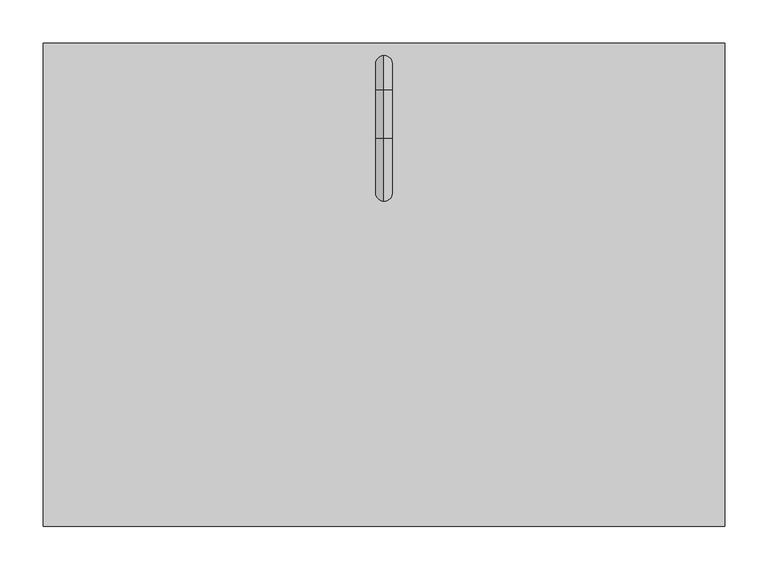
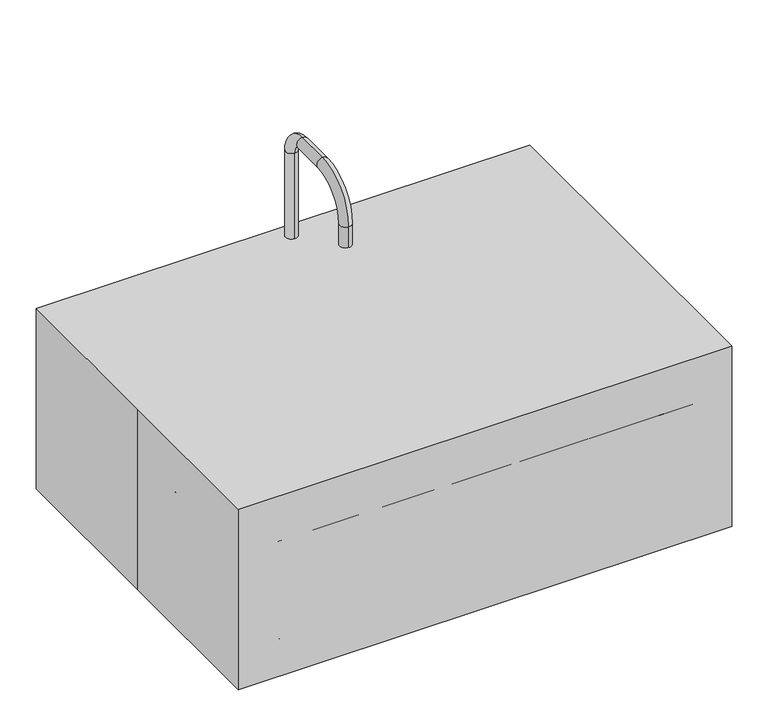
"""IFC4 building model written with IfcOpenShell, lengths in millimetres: proxy geometry, CS200 - Sink, SS, Single Compartment, 12x28x16 ID : CS200 - Sink, SS, Single Compartment, 12x28x16 ID."""

from ifc_helpers import new_model, si_unit, point, frame, frame_2d, origin, origin_with_axes, origin_2d, place, context, project, spatial, polyline, circle_curve, ellipse_curve, trimmed, segment, composite_curve, outline, extrude, source, transform, mapped, element, save
from ifc_brep_helpers import plane_surface, cylinder_surface, revolved_surface, advanced_brep


def specialty_equipment_f0ebf2b9(model_context):
    return source(origin(), model_context, "Body", "SolidModel", [
        extrude(outline(composite_curve([segment(trimmed(circle_curve(frame_2d((292.1, 168.275)), 25.4), [point((292.1, 193.675))], [point((317.5, 168.275))], False, "CARTESIAN"), True, "CONTINUOUS"), segment(polyline([(317.5, 168.275), (317.5, -177.8)]), True, "CONTINUOUS"), segment(trimmed(circle_curve(frame_2d((292.1, -177.8)), 25.4), [point((317.5, -177.8))], [point((292.1, -203.2))], False, "CARTESIAN"), True, "CONTINUOUS"), segment(polyline([(292.1, -203.2), (-292.1000001, -203.2)]), True, "CONTINUOUS"), segment(trimmed(circle_curve(frame_2d((-292.1000001, -177.8)), 25.4), [point((-292.1000001, -203.2))], [point((-317.5000001, -177.8))], False, "CARTESIAN"), True, "CONTINUOUS"), segment(polyline([(-317.5000001, -177.8), (-317.5000001, 168.275)]), True, "CONTINUOUS"), segment(trimmed(circle_curve(frame_2d((-292.1000001, 168.275)), 25.4), [point((-317.5000001, 168.275))], [point((-292.1000001, 193.675))], False, "CARTESIAN"), True, "CONTINUOUS"), segment(polyline([(-292.1000001, 193.675), (292.1, 193.675)]), True, "CONTINUOUS")], self_intersect=False), holes=[composite_curve([segment(trimmed(circle_curve(origin_2d(), 25.4), [point((-25.4, 0.0))], [point((25.4, 0.0))], True, "CARTESIAN"), True, "CONTINUOUS"), segment(trimmed(circle_curve(origin_2d(), 25.4), [point((25.4, 0.0))], [point((-25.4, 0.0))], True, "CARTESIAN"), True, "CONTINUOUS")], self_intersect=False)]), origin_with_axes(), (0.0, 0.0, 1.0), 9.525),
        extrude(outline(polyline([(-393.7, 279.4), (393.7, 279.4), (393.7, -279.4), (-393.7, -279.4), (-393.7, 0.0), (-393.7, 279.4)])), origin_with_axes(), (0.0, 0.0, 1.0), 304.8),
        extrude(outline(composite_curve([segment(trimmed(circle_curve(frame_2d((82.55, 260.35)), 19.05), [point((82.55, 279.4))], [point((82.55, 241.3))], False, "CARTESIAN"), True, "CONTINUOUS"), segment(polyline([(82.55, 241.3), (-82.55, 241.3)]), True, "CONTINUOUS"), segment(trimmed(circle_curve(frame_2d((-82.55, 260.35)), 19.05), [point((-82.55, 241.3))], [point((-82.55, 279.4))], False, "CARTESIAN"), True, "CONTINUOUS"), segment(polyline([(-82.55, 279.4), (82.55, 279.4)]), True, "CONTINUOUS")], self_intersect=False), holes=[composite_curve([segment(trimmed(circle_curve(frame_2d((0.0, 255.5875)), 9.525), [point((-9.525, 255.5875))], [point((9.525, 255.5875))], True, "CARTESIAN"), True, "CONTINUOUS"), segment(trimmed(circle_curve(frame_2d((0.0, 255.5875)), 9.525), [point((9.525, 255.5875))], [point((-9.525, 255.5875))], True, "CARTESIAN"), True, "CONTINUOUS")], self_intersect=False)]), frame((0.0, 0.0, 228.6), z_axis=(0.0, 0.0, 1.0), x_axis=(1.0, 0.0, 0.0)), (0.0, 0.0, 1.0), 12.7),
        extrude(outline(composite_curve([segment(trimmed(circle_curve(frame_2d((-1e-07, 255.5875)), 12.7), [point((-12.7000001, 255.5875))], [point((12.6999999, 255.5875))], False, "CARTESIAN"), True, "CONTINUOUS"), segment(trimmed(circle_curve(frame_2d((-1e-07, 255.5875)), 12.7), [point((12.6999999, 255.5875))], [point((-12.7000001, 255.5875))], False, "CARTESIAN"), True, "CONTINUOUS")], self_intersect=False), holes=[composite_curve([segment(trimmed(circle_curve(frame_2d((-1e-07, 255.5875)), 9.525), [point((-9.5250001, 255.5875))], [point((9.5249999, 255.5875))], True, "CARTESIAN"), True, "CONTINUOUS"), segment(trimmed(circle_curve(frame_2d((-1e-07, 255.5875)), 9.525), [point((9.5249999, 255.5875))], [point((-9.5250001, 255.5875))], True, "CARTESIAN"), True, "CONTINUOUS")], self_intersect=False)]), frame((0.0, 0.0, 241.3), z_axis=(0.0, 0.0, 1.0), x_axis=(1.0, 0.0, 0.0)), (0.0, 0.0, 1.0), 12.7),
        advanced_brep(
        [(-1e-07, 265.1125, 228.6), (-1e-07, 246.0625, 228.6), (-1e-07, 265.1125, 449.2625), (-1e-07, 246.0625, 449.2625), (-1e-07, 225.425, 469.9), (-1e-07, 225.425, 488.95), (-1e-07, 169.8625, 488.95), (-1e-07, 169.8625, 469.9), (-1e-07, 115.8875, 415.925), (-1e-07, 96.8375, 415.925), (-1e-07, 96.8375, 381.0), (-1e-07, 115.8875, 381.0)],
        [
            (0, 1, circle_curve(frame((-1e-07, 255.5875, 228.6), z_axis=(0.0, 0.0, -1.0), x_axis=(0.0, -1.0, 0.0)), 9.525)),
            (1, 0, circle_curve(frame((-1e-07, 255.5875, 228.6), z_axis=(0.0, 0.0, -1.0), x_axis=(0.0, -1.0, 0.0)), 9.525)),
            (0, 2),
            (2, 3, circle_curve(frame((-1e-07, 255.5875, 449.2625), z_axis=(0.0, 0.0, -1.0), x_axis=(0.0, -1.0, 0.0)), 9.525)),
            (3, 1),
            (3, 2, circle_curve(frame((-1e-07, 255.5875, 449.2625), z_axis=(0.0, 0.0, -1.0), x_axis=(0.0, -1.0, 0.0)), 9.525)),
            (4, 3, circle_curve(frame((-1e-07, 225.425, 449.2625), z_axis=(-1.0, 0.0, 0.0), x_axis=(0.0, 1.0, 0.0)), 20.6375)),
            (2, 5, circle_curve(frame((-1e-07, 225.425, 449.2625), z_axis=(1.0, 0.0, 0.0), x_axis=(0.0, 1.0, 0.0)), 39.6875)),
            (5, 4, circle_curve(frame((-1e-07, 225.425, 479.425), z_axis=(0.0, 1.0, 0.0), x_axis=(0.0, 0.0, -1.0)), 9.525)),
            (4, 5, circle_curve(frame((-1e-07, 225.425, 479.425), z_axis=(0.0, 1.0, 0.0), x_axis=(0.0, 0.0, -1.0)), 9.525)),
            (5, 6),
            (6, 7, circle_curve(frame((-1e-07, 169.8625, 479.425), z_axis=(0.0, 1.0, 0.0), x_axis=(0.0, 0.0, -1.0)), 9.525)),
            (7, 4),
            (7, 6, circle_curve(frame((-1e-07, 169.8625, 479.425), z_axis=(0.0, 1.0, 0.0), x_axis=(0.0, 0.0, -1.0)), 9.525)),
            (8, 7, circle_curve(frame((-1e-07, 169.8625, 415.925), z_axis=(-1.0, 0.0, 0.0), x_axis=(0.0, 0.0, 1.0)), 53.975)),
            (6, 9, circle_curve(frame((-1e-07, 169.8625, 415.925), z_axis=(1.0, 0.0, 0.0), x_axis=(0.0, 0.0, 1.0)), 73.025)),
            (9, 8, circle_curve(frame((-1e-07, 106.3625, 415.925), z_axis=(0.0, 0.0, 1.0), x_axis=(0.0, 1.0, 0.0)), 9.525)),
            (8, 9, circle_curve(frame((-1e-07, 106.3625, 415.925), z_axis=(0.0, 0.0, 1.0), x_axis=(0.0, 1.0, 0.0)), 9.525)),
            (10, 11, circle_curve(frame((-1e-07, 106.3625, 381.0), z_axis=(0.0, 0.0, -1.0), x_axis=(0.0, 1.0, 0.0)), 9.525)),
            (11, 10, circle_curve(frame((-1e-07, 106.3625, 381.0), z_axis=(0.0, 0.0, -1.0), x_axis=(0.0, 1.0, 0.0)), 9.525)),
            (9, 10),
            (11, 8),
        ],
        [
            plane_surface(frame((-1e-07, 246.0625, 228.6), z_axis=(0.0, 0.0, -1.0), x_axis=(1.0, 0.0, 0.0))),
            cylinder_surface(frame((-1e-07, 255.5875, 228.6), z_axis=(0.0, 0.0, -1.0), x_axis=(0.0, -1.0, 0.0)), 9.525),
            revolved_surface(trimmed(ellipse_curve(frame((-1e-07, 255.5875, 449.2625), z_axis=(0.0, 0.0, -1.0), x_axis=(0.0, -1.0, 0.0)), 9.525, 9.525), [point((-1e-07, 265.1125, 449.2625))], [point((-1e-07, 246.0625, 449.2625))], True, "CARTESIAN"), (-1e-07, 225.425, 449.2625), (1.0, 0.0, 0.0)),
            revolved_surface(trimmed(ellipse_curve(frame((-1e-07, 255.5875, 449.2625), z_axis=(0.0, 0.0, -1.0), x_axis=(0.0, -1.0, 0.0)), 9.525, 9.525), [point((-1e-07, 246.0625, 449.2625))], [point((-1e-07, 265.1125, 449.2625))], True, "CARTESIAN"), (-1e-07, 225.425, 449.2625), (1.0, 0.0, 0.0)),
            cylinder_surface(frame((-1e-07, 225.425, 479.425), z_axis=(0.0, 1.0, 0.0), x_axis=(0.0, 0.0, -1.0)), 9.525),
            revolved_surface(trimmed(ellipse_curve(frame((-1e-07, 169.8625, 479.425), z_axis=(0.0, 1.0, 0.0), x_axis=(0.0, 0.0, -1.0)), 9.525, 9.525), [point((-1e-07, 169.8625, 488.95))], [point((-1e-07, 169.8625, 469.9))], True, "CARTESIAN"), (-1e-07, 169.8625, 415.925), (1.0, 0.0, 0.0)),
            revolved_surface(trimmed(ellipse_curve(frame((-1e-07, 169.8625, 479.425), z_axis=(0.0, 1.0, 0.0), x_axis=(0.0, 0.0, -1.0)), 9.525, 9.525), [point((-1e-07, 169.8625, 469.9))], [point((-1e-07, 169.8625, 488.95))], True, "CARTESIAN"), (-1e-07, 169.8625, 415.925), (1.0, 0.0, 0.0)),
            plane_surface(frame((-1e-07, 96.8375, 381.0), z_axis=(0.0, 0.0, -1.0), x_axis=(-1.0, 0.0, 0.0))),
            cylinder_surface(frame((-1e-07, 106.3625, 415.925), z_axis=(0.0, 0.0, 1.0), x_axis=(0.0, 1.0, 0.0)), 9.525),
        ],
        [
            (0, [[1, 2]]),
            (1, [[-1, 3, 4, 5]]),
            (1, [[-2, -5, 6, -3]]),
            (2, [[7, -4, 8, 9]]),
            (3, [[-8, -6, -7, 10]]),
            (4, [[-9, 11, 12, 13]]),
            (4, [[-10, -13, 14, -11]]),
            (5, [[15, -12, 16, 17]]),
            (6, [[-16, -14, -15, 18]]),
            (7, [[19, 20]]),
            (8, [[-17, 21, -20, 22]]),
            (8, [[-18, -22, -19, -21]]),
        ],
    ),
        extrude(outline(composite_curve([segment(trimmed(circle_curve(frame_2d((-57.15, 260.35)), 19.05), [point((-76.2, 260.35))], [point((-38.1, 260.35))], False, "CARTESIAN"), True, "CONTINUOUS"), segment(trimmed(circle_curve(frame_2d((-57.15, 260.35)), 19.05), [point((-38.1, 260.35))], [point((-76.2, 260.35))], False, "CARTESIAN"), True, "CONTINUOUS")], self_intersect=False)), frame((0.0, 0.0, 241.3), z_axis=(0.0, 0.0, 1.0), x_axis=(1.0, 0.0, 0.0)), (0.0, 0.0, 1.0), 50.8),
        extrude(outline(composite_curve([segment(trimmed(circle_curve(frame_2d((57.15, 260.35)), 19.05), [point((38.1, 260.35))], [point((76.2, 260.35))], False, "CARTESIAN"), True, "CONTINUOUS"), segment(trimmed(circle_curve(frame_2d((57.15, 260.35)), 19.05), [point((76.2, 260.35))], [point((38.1, 260.35))], False, "CARTESIAN"), True, "CONTINUOUS")], self_intersect=False)), frame((0.0, 0.0, 241.3), z_axis=(0.0, 0.0, 1.0), x_axis=(1.0, 0.0, 0.0)), (0.0, 0.0, 1.0), 50.8),
        advanced_brep(
        [(-292.1000001, 238.125, 0.0), (-292.1000001, 238.125, 215.9), (292.1, 238.125, 215.9), (292.1, 238.125, 0.0), (-292.1000001, 193.675, 0.0), (292.1, 193.675, 0.0), (-292.1000001, 193.675, 9.525), (292.1, 193.675, 9.525), (-292.1000001, 196.2634182, 9.525), (292.1, 196.2634182, 9.525), (-292.1000001, 215.2409272, 26.9146831), (292.1, 215.2409272, 26.9146831), (-292.1000001, 231.775, 215.9), (292.1, 231.775, 215.9), (361.95, 168.275, 0.0), (361.95, 168.275, 215.9), (317.5, 168.275, 0.0), (317.5, 168.275, 9.525), (320.0884182, 168.275, 9.525), (339.0659272, 168.275, 26.9146831), (355.6, 168.275, 215.9), (361.95, -177.8, 215.9), (361.95, -177.8, 0.0), (317.5, -177.8, 0.0), (317.5, -177.8, 9.525), (320.0884182, -177.8, 9.525), (339.0659272, -177.8, 26.9146831), (355.6, -177.8, 215.9), (292.1, -247.65, 0.0), (292.1, -247.65, 215.9), (292.1, -203.2, 0.0), (292.1, -203.2, 9.525), (292.1, -205.7884182, 9.525), (292.1, -224.7659272, 26.9146831), (292.1, -241.3, 215.9), (-292.1000001, -247.65, 215.9), (-292.1000001, -247.65, 0.0), (-292.1000001, -203.2, 0.0), (-292.1000001, -203.2, 9.525), (-292.1000001, -205.7884182, 9.525), (-292.1000001, -224.7659272, 26.9146831), (-292.1000001, -241.3, 215.9), (-361.9500001, -177.8, 0.0), (-361.9500001, -177.8, 215.9), (-317.5000001, -177.8, 0.0), (-317.5000001, -177.8, 9.525), (-320.0884183, -177.8, 9.525), (-339.0659273, -177.8, 26.9146831), (-355.6000001, -177.8, 215.9), (-361.9500001, 168.275, 215.9), (-361.9500001, 168.275, 0.0), (-317.5000001, 168.275, 0.0), (-317.5000001, 168.275, 9.525), (-320.0884183, 168.275, 9.525), (-339.0659273, 168.275, 26.9146831), (-355.6000001, 168.275, 215.9)],
        [
            (0, 1),
            (1, 2),
            (2, 3),
            (3, 0),
            (4, 0),
            (3, 5),
            (5, 4),
            (6, 4),
            (5, 7),
            (7, 6),
            (8, 6),
            (7, 9),
            (9, 8),
            (10, 8, circle_curve(frame((-292.1000001, 196.2634182, 28.575), z_axis=(-1.0, 0.0, 0.0), x_axis=(0.0, 1.0, 0.0)), 19.05)),
            (9, 11, circle_curve(frame((292.1, 196.2634182, 28.575), z_axis=(1.0, 0.0, 0.0), x_axis=(0.0, 1.0, 0.0)), 19.05)),
            (11, 10),
            (12, 10),
            (11, 13),
            (13, 12),
            (1, 12),
            (13, 2),
            (14, 3, circle_curve(frame((292.1, 168.275, 0.0), z_axis=(0.0, 0.0, 1.0), x_axis=(0.0, 1.0, 0.0)), 69.85)),
            (2, 15, circle_curve(frame((292.1, 168.275, 215.9), z_axis=(0.0, 0.0, -1.0), x_axis=(0.0, 1.0, 0.0)), 69.85)),
            (15, 14),
            (16, 5, circle_curve(frame((292.1, 168.275, 0.0), z_axis=(0.0, 0.0, 1.0), x_axis=(0.0, 1.0, 0.0)), 25.4)),
            (14, 16),
            (17, 7, circle_curve(frame((292.1, 168.275, 9.525), z_axis=(0.0, 0.0, 1.0), x_axis=(0.0, 1.0, 0.0)), 25.4)),
            (16, 17),
            (18, 9, circle_curve(frame((292.1, 168.275, 9.525), z_axis=(0.0, 0.0, 1.0), x_axis=(0.0, 1.0, 0.0)), 27.9884182)),
            (17, 18),
            (19, 11, circle_curve(frame((292.1, 168.275, 26.9146831), z_axis=(0.0, 0.0, 1.0), x_axis=(0.0, 1.0, 0.0)), 46.9659272)),
            (18, 19, circle_curve(frame((320.0884182, 168.275, 28.575), z_axis=(0.0, -1.0, 0.0), x_axis=(1.0, 0.0, 0.0)), 19.05)),
            (20, 13, circle_curve(frame((292.1, 168.275, 215.9), z_axis=(0.0, 0.0, 1.0), x_axis=(0.0, 1.0, 0.0)), 63.5)),
            (19, 20),
            (20, 15),
            (15, 21),
            (21, 22),
            (22, 14),
            (22, 23),
            (23, 16),
            (23, 24),
            (24, 17),
            (24, 25),
            (25, 18),
            (25, 26, circle_curve(frame((320.0884182, -177.8, 28.575), z_axis=(0.0, -1.0, 0.0), x_axis=(1.0, 0.0, 0.0)), 19.05)),
            (26, 19),
            (26, 27),
            (27, 20),
            (27, 21),
            (28, 22, circle_curve(frame((292.1, -177.8, 0.0), z_axis=(0.0, 0.0, 1.0), x_axis=(1.0, 0.0, 0.0)), 69.85)),
            (21, 29, circle_curve(frame((292.1, -177.8, 215.9), z_axis=(0.0, 0.0, -1.0), x_axis=(1.0, 0.0, 0.0)), 69.85)),
            (29, 28),
            (30, 23, circle_curve(frame((292.1, -177.8, 0.0), z_axis=(0.0, 0.0, 1.0), x_axis=(1.0, 0.0, 0.0)), 25.4)),
            (28, 30),
            (31, 24, circle_curve(frame((292.1, -177.8, 9.525), z_axis=(0.0, 0.0, 1.0), x_axis=(1.0, 0.0, 0.0)), 25.4)),
            (30, 31),
            (32, 25, circle_curve(frame((292.1, -177.8, 9.525), z_axis=(0.0, 0.0, 1.0), x_axis=(1.0, 0.0, 0.0)), 27.9884182)),
            (31, 32),
            (33, 26, circle_curve(frame((292.1, -177.8, 26.9146831), z_axis=(0.0, 0.0, 1.0), x_axis=(1.0, 0.0, 0.0)), 46.9659272)),
            (32, 33, circle_curve(frame((292.1, -205.7884182, 28.575), z_axis=(-1.0, 0.0, 0.0), x_axis=(0.0, -1.0, 0.0)), 19.05)),
            (34, 27, circle_curve(frame((292.1, -177.8, 215.9), z_axis=(0.0, 0.0, 1.0), x_axis=(1.0, 0.0, 0.0)), 63.5)),
            (33, 34),
            (34, 29),
            (29, 35),
            (35, 36),
            (36, 28),
            (36, 37),
            (37, 30),
            (37, 38),
            (38, 31),
            (38, 39),
            (39, 32),
            (39, 40, circle_curve(frame((-292.1000001, -205.7884182, 28.575), z_axis=(-1.0, 0.0, 0.0), x_axis=(0.0, -1.0, 0.0)), 19.05)),
            (40, 33),
            (40, 41),
            (41, 34),
            (41, 35),
            (42, 36, circle_curve(frame((-292.1000001, -177.8, 0.0), z_axis=(0.0, 0.0, 1.0), x_axis=(0.0, -1.0, 0.0)), 69.85)),
            (35, 43, circle_curve(frame((-292.1000001, -177.8, 215.9), z_axis=(0.0, 0.0, -1.0), x_axis=(0.0, -1.0, 0.0)), 69.85)),
            (43, 42),
            (44, 37, circle_curve(frame((-292.1000001, -177.8, 0.0), z_axis=(0.0, 0.0, 1.0), x_axis=(0.0, -1.0, 0.0)), 25.4)),
            (42, 44),
            (45, 38, circle_curve(frame((-292.1000001, -177.8, 9.525), z_axis=(0.0, 0.0, 1.0), x_axis=(0.0, -1.0, 0.0)), 25.4)),
            (44, 45),
            (46, 39, circle_curve(frame((-292.1000001, -177.8, 9.525), z_axis=(0.0, 0.0, 1.0), x_axis=(0.0, -1.0, 0.0)), 27.9884182)),
            (45, 46),
            (47, 40, circle_curve(frame((-292.1000001, -177.8, 26.9146831), z_axis=(0.0, 0.0, 1.0), x_axis=(0.0, -1.0, 0.0)), 46.9659272)),
            (46, 47, circle_curve(frame((-320.0884183, -177.8, 28.575), z_axis=(0.0, 1.0, 0.0), x_axis=(-1.0, 0.0, 0.0)), 19.05)),
            (48, 41, circle_curve(frame((-292.1000001, -177.8, 215.9), z_axis=(0.0, 0.0, 1.0), x_axis=(0.0, -1.0, 0.0)), 63.5)),
            (47, 48),
            (48, 43),
            (43, 49),
            (49, 50),
            (50, 42),
            (50, 51),
            (51, 44),
            (51, 52),
            (52, 45),
            (52, 53),
            (53, 46),
            (53, 54, circle_curve(frame((-320.0884183, 168.275, 28.575), z_axis=(0.0, 1.0, 0.0), x_axis=(-1.0, 0.0, 0.0)), 19.05)),
            (54, 47),
            (54, 55),
            (55, 48),
            (55, 49),
            (0, 50, circle_curve(frame((-292.1000001, 168.275, 0.0), z_axis=(0.0, 0.0, 1.0), x_axis=(-1.0, 0.0, 0.0)), 69.85)),
            (49, 1, circle_curve(frame((-292.1000001, 168.275, 215.9), z_axis=(0.0, 0.0, -1.0), x_axis=(-1.0, 0.0, 0.0)), 69.85)),
            (4, 51, circle_curve(frame((-292.1000001, 168.275, 0.0), z_axis=(0.0, 0.0, 1.0), x_axis=(-1.0, 0.0, 0.0)), 25.4)),
            (6, 52, circle_curve(frame((-292.1000001, 168.275, 9.525), z_axis=(0.0, 0.0, 1.0), x_axis=(-1.0, 0.0, 0.0)), 25.4)),
            (8, 53, circle_curve(frame((-292.1000001, 168.275, 9.525), z_axis=(0.0, 0.0, 1.0), x_axis=(-1.0, 0.0, 0.0)), 27.9884182)),
            (10, 54, circle_curve(frame((-292.1000001, 168.275, 26.9146831), z_axis=(0.0, 0.0, 1.0), x_axis=(-1.0, 0.0, 0.0)), 46.9659272)),
            (12, 55, circle_curve(frame((-292.1000001, 168.275, 215.9), z_axis=(0.0, 0.0, 1.0), x_axis=(-1.0, 0.0, 0.0)), 63.5)),
        ],
        [
            plane_surface(frame((-292.1000001, 238.125, 215.9), z_axis=(0.0, 1.0, 0.0), x_axis=(1.0, 0.0, 0.0))),
            plane_surface(frame((-292.1000001, 238.125, 0.0), z_axis=(0.0, 0.0, -1.0), x_axis=(1.0, 0.0, 0.0))),
            plane_surface(frame((-292.1000001, 193.675, 0.0), z_axis=(0.0, -1.0, 0.0), x_axis=(1.0, 0.0, 0.0))),
            plane_surface(frame((-292.1000001, 193.675, 9.525), z_axis=(0.0, 0.0, 1.0), x_axis=(1.0, 0.0, 0.0))),
            revolved_surface(polyline([(292.1, 215.3134182, 28.575), (-292.1000001, 215.3134182, 28.575)]), (-292.1000001, 196.2634182, 28.575), (1.0, 0.0, 0.0)),
            plane_surface(frame((-292.1000001, 215.2409272, 26.9146831), z_axis=(0.0, -0.9961946980917442, 0.08715574274767357), x_axis=(1.0, 0.0, 0.0))),
            plane_surface(frame((-292.1000001, 231.775, 215.9), z_axis=(0.0, 0.0, 1.0), x_axis=(1.0, 0.0, 0.0))),
            cylinder_surface(frame((292.1, 168.275, -647.7), z_axis=(0.0, 0.0, -1.0), x_axis=(0.0, 1.0, 0.0)), 69.85),
            plane_surface(frame((292.1, 168.275, 0.0), z_axis=(0.0, 0.0, -1.0), x_axis=(0.0, 1.0, 0.0))),
            revolved_surface(polyline([(292.1, 193.675, 0.0), (292.1, 193.675, 9.524999999999977)]), (292.1, 168.275, -647.7), (0.0, 0.0, -1.0)),
            plane_surface(frame((292.1, 168.275, 9.525), z_axis=(0.0, 0.0, 1.0), x_axis=(0.0, 1.0, 0.0))),
            revolved_surface(trimmed(ellipse_curve(frame((292.1, 196.2634182, 28.575), z_axis=(1.0, 0.0, 0.0), x_axis=(0.0, 1.0, 0.0)), 19.05, 19.05), [point((292.1, 196.2634182, 9.525))], [point((292.1, 215.2409272, 26.9146831))], True, "CARTESIAN"), (292.1, 168.275, -647.7), (0.0, 0.0, -1.0)),
            revolved_surface(polyline([(292.1, 215.2409272, 26.9146831), (292.1, 231.775, 215.9)]), (292.1, 168.275, -647.7), (0.0, 0.0, -1.0)),
            plane_surface(frame((292.1, 168.275, 215.9), z_axis=(0.0, 0.0, 1.0), x_axis=(0.0, 1.0, 0.0))),
            plane_surface(frame((361.95, 168.275, 215.9), z_axis=(1.0, 0.0, 0.0), x_axis=(0.0, -1.0, 0.0))),
            plane_surface(frame((361.95, 168.275, 0.0), z_axis=(0.0, 0.0, -1.0), x_axis=(0.0, -1.0, 0.0))),
            plane_surface(frame((317.5, 168.275, 0.0), z_axis=(-1.0, 0.0, 0.0), x_axis=(0.0, -1.0, 0.0))),
            plane_surface(frame((317.5, 168.275, 9.525), z_axis=(0.0, 0.0, 1.0), x_axis=(0.0, -1.0, 0.0))),
            revolved_surface(polyline([(339.1384182, -177.80000000000004, 28.575), (339.1384182, 168.275, 28.575)]), (320.0884182, 168.275, 28.575), (0.0, -1.0, 0.0)),
            plane_surface(frame((339.0659272, 168.275, 26.9146831), z_axis=(-0.9961946980917442, 0.0, 0.08715574274767357), x_axis=(0.0, -1.0, 0.0))),
            plane_surface(frame((355.6, 168.275, 215.9), z_axis=(0.0, 0.0, 1.0), x_axis=(0.0, -1.0, 0.0))),
            cylinder_surface(frame((292.1, -177.8, -647.7), z_axis=(0.0, 0.0, -1.0), x_axis=(1.0, 0.0, 0.0)), 69.85),
            plane_surface(frame((292.1, -177.8, 0.0), z_axis=(0.0, 0.0, -1.0), x_axis=(1.0, 0.0, 0.0))),
            revolved_surface(polyline([(317.5, -177.8, 0.0), (317.5, -177.8, 9.524999999999977)]), (292.1, -177.8, -647.7), (0.0, 0.0, -1.0)),
            plane_surface(frame((292.1, -177.8, 9.525), z_axis=(0.0, 0.0, 1.0), x_axis=(1.0, 0.0, 0.0))),
            revolved_surface(trimmed(ellipse_curve(frame((320.0884182, -177.8, 28.575), z_axis=(0.0, -1.0, 0.0), x_axis=(1.0, 0.0, 0.0)), 19.05, 19.05), [point((320.0884182, -177.8, 9.525))], [point((339.0659272, -177.8, 26.9146831))], True, "CARTESIAN"), (292.1, -177.8, -647.7), (0.0, 0.0, -1.0)),
            revolved_surface(polyline([(339.0659272, -177.8, 26.9146831), (355.6, -177.8, 215.9)]), (292.1, -177.8, -647.7), (0.0, 0.0, -1.0)),
            plane_surface(frame((292.1, -177.8, 215.9), z_axis=(0.0, 0.0, 1.0), x_axis=(1.0, 0.0, 0.0))),
            plane_surface(frame((292.1, -247.65, 215.9), z_axis=(0.0, -1.0, 0.0), x_axis=(-1.0, 0.0, 0.0))),
            plane_surface(frame((292.1, -247.65, 0.0), z_axis=(0.0, 0.0, -1.0), x_axis=(-1.0, 0.0, 0.0))),
            plane_surface(frame((292.1, -203.2, 0.0), z_axis=(0.0, 1.0, 0.0), x_axis=(-1.0, 0.0, 0.0))),
            plane_surface(frame((292.1, -203.2, 9.525), z_axis=(0.0, 0.0, 1.0), x_axis=(-1.0, 0.0, 0.0))),
            revolved_surface(polyline([(-292.1000001, -224.8384182, 28.575), (292.1, -224.8384182, 28.575)]), (292.1, -205.7884182, 28.575), (-1.0, 0.0, 0.0)),
            plane_surface(frame((292.1, -224.7659272, 26.9146831), z_axis=(0.0, 0.9961946980917442, 0.08715574274767357), x_axis=(-1.0, 0.0, 0.0))),
            plane_surface(frame((292.1, -241.3, 215.9), z_axis=(0.0, 0.0, 1.0), x_axis=(-1.0, 0.0, 0.0))),
            cylinder_surface(frame((-292.1000001, -177.8, -647.7), z_axis=(0.0, 0.0, -1.0), x_axis=(0.0, -1.0, 0.0)), 69.85),
            plane_surface(frame((-292.1000001, -177.8, 0.0), z_axis=(0.0, 0.0, -1.0), x_axis=(0.0, -1.0, 0.0))),
            revolved_surface(polyline([(-292.1000001, -203.20000000000002, 0.0), (-292.1000001, -203.20000000000002, 9.524999999999977)]), (-292.1000001, -177.8, -647.7), (0.0, 0.0, -1.0)),
            plane_surface(frame((-292.1000001, -177.8, 9.525), z_axis=(0.0, 0.0, 1.0), x_axis=(0.0, -1.0, 0.0))),
            revolved_surface(trimmed(ellipse_curve(frame((-292.1000001, -205.7884182, 28.575), z_axis=(-1.0, 0.0, 0.0), x_axis=(0.0, -1.0, 0.0)), 19.05, 19.05), [point((-292.1000001, -205.7884182, 9.525))], [point((-292.1000001, -224.7659272, 26.9146831))], True, "CARTESIAN"), (-292.1000001, -177.8, -647.7), (0.0, 0.0, -1.0)),
            revolved_surface(polyline([(-292.1000001, -224.7659272, 26.9146831), (-292.1000001, -241.3, 215.9)]), (-292.1000001, -177.8, -647.7), (0.0, 0.0, -1.0)),
            plane_surface(frame((-292.1000001, -177.8, 215.9), z_axis=(0.0, 0.0, 1.0), x_axis=(0.0, -1.0, 0.0))),
            plane_surface(frame((-361.9500001, -177.8, 215.9), z_axis=(-1.0, 0.0, 0.0), x_axis=(0.0, 1.0, 0.0))),
            plane_surface(frame((-361.9500001, -177.8, 0.0), z_axis=(0.0, 0.0, -1.0), x_axis=(0.0, 1.0, 0.0))),
            plane_surface(frame((-317.5000001, -177.8, 0.0), z_axis=(1.0, 0.0, 0.0), x_axis=(0.0, 1.0, 0.0))),
            plane_surface(frame((-317.5000001, -177.8, 9.525), z_axis=(0.0, 0.0, 1.0), x_axis=(0.0, 1.0, 0.0))),
            revolved_surface(polyline([(-339.1384183, 168.27500000000003, 28.575), (-339.1384183, -177.8, 28.575)]), (-320.0884183, -177.8, 28.575), (0.0, 1.0, 0.0)),
            plane_surface(frame((-339.0659273, -177.8, 26.9146831), z_axis=(0.9961946980917442, 0.0, 0.08715574274767357), x_axis=(0.0, 1.0, 0.0))),
            plane_surface(frame((-355.6000001, -177.8, 215.9), z_axis=(0.0, 0.0, 1.0), x_axis=(0.0, 1.0, 0.0))),
            cylinder_surface(frame((-292.1000001, 168.275, -647.7), z_axis=(0.0, 0.0, -1.0), x_axis=(-1.0, 0.0, 0.0)), 69.85),
            plane_surface(frame((-292.1000001, 168.275, 0.0), z_axis=(0.0, 0.0, -1.0), x_axis=(-1.0, 0.0, 0.0))),
            revolved_surface(polyline([(-317.50000009999997, 168.275, 0.0), (-317.50000009999997, 168.275, 9.524999999999977)]), (-292.1000001, 168.275, -647.7), (0.0, 0.0, -1.0)),
            plane_surface(frame((-292.1000001, 168.275, 9.525), z_axis=(0.0, 0.0, 1.0), x_axis=(-1.0, 0.0, 0.0))),
            revolved_surface(trimmed(ellipse_curve(frame((-320.0884183, 168.275, 28.575), z_axis=(0.0, 1.0, 0.0), x_axis=(-1.0, 0.0, 0.0)), 19.05, 19.05), [point((-320.0884183, 168.275, 9.525))], [point((-339.0659273, 168.275, 26.9146831))], True, "CARTESIAN"), (-292.1000001, 168.275, -647.7), (0.0, 0.0, -1.0)),
            revolved_surface(polyline([(-339.0659273, 168.275, 26.9146831), (-355.6000001, 168.275, 215.9)]), (-292.1000001, 168.275, -647.7), (0.0, 0.0, -1.0)),
            plane_surface(frame((-292.1000001, 168.275, 215.9), z_axis=(0.0, 0.0, 1.0), x_axis=(-1.0, 0.0, 0.0))),
        ],
        [
            (0, [[1, 2, 3, 4]]),
            (1, [[5, -4, 6, 7]]),
            (2, [[8, -7, 9, 10]]),
            (3, [[11, -10, 12, 13]]),
            (4, [[14, -13, 15, 16]]),
            (5, [[17, -16, 18, 19]]),
            (6, [[20, -19, 21, -2]]),
            (7, [[22, -3, 23, 24]]),
            (8, [[25, -6, -22, 26]]),
            (9, [[27, -9, -25, 28]]),
            (10, [[29, -12, -27, 30]]),
            (11, [[31, -15, -29, 32]]),
            (12, [[33, -18, -31, 34]]),
            (13, [[-23, -21, -33, 35]]),
            (14, [[-24, 36, 37, 38]]),
            (15, [[-26, -38, 39, 40]]),
            (16, [[-28, -40, 41, 42]]),
            (17, [[-30, -42, 43, 44]]),
            (18, [[-32, -44, 45, 46]]),
            (19, [[-34, -46, 47, 48]]),
            (20, [[-35, -48, 49, -36]]),
            (21, [[50, -37, 51, 52]]),
            (22, [[53, -39, -50, 54]]),
            (23, [[55, -41, -53, 56]]),
            (24, [[57, -43, -55, 58]]),
            (25, [[59, -45, -57, 60]]),
            (26, [[61, -47, -59, 62]]),
            (27, [[-51, -49, -61, 63]]),
            (28, [[-52, 64, 65, 66]]),
            (29, [[-54, -66, 67, 68]]),
            (30, [[-56, -68, 69, 70]]),
            (31, [[-58, -70, 71, 72]]),
            (32, [[-60, -72, 73, 74]]),
            (33, [[-62, -74, 75, 76]]),
            (34, [[-63, -76, 77, -64]]),
            (35, [[78, -65, 79, 80]]),
            (36, [[81, -67, -78, 82]]),
            (37, [[83, -69, -81, 84]]),
            (38, [[85, -71, -83, 86]]),
            (39, [[87, -73, -85, 88]]),
            (40, [[89, -75, -87, 90]]),
            (41, [[-79, -77, -89, 91]]),
            (42, [[-80, 92, 93, 94]]),
            (43, [[-82, -94, 95, 96]]),
            (44, [[-84, -96, 97, 98]]),
            (45, [[-86, -98, 99, 100]]),
            (46, [[-88, -100, 101, 102]]),
            (47, [[-90, -102, 103, 104]]),
            (48, [[-91, -104, 105, -92]]),
            (49, [[106, -93, 107, -1]]),
            (50, [[108, -95, -106, -5]]),
            (51, [[109, -97, -108, -8]]),
            (52, [[110, -99, -109, -11]]),
            (53, [[111, -101, -110, -14]]),
            (54, [[112, -103, -111, -17]]),
            (55, [[-107, -105, -112, -20]]),
        ],
    ),
        extrude(outline(composite_curve([segment(trimmed(circle_curve(frame_2d((-330.2, -215.9)), 63.5), [point((-330.2, -279.4))], [point((-393.7, -215.9))], False, "CARTESIAN"), True, "CONTINUOUS"), segment(polyline([(-393.7, -215.9), (-393.7, 215.9)]), True, "CONTINUOUS"), segment(trimmed(circle_curve(frame_2d((-330.2, 215.9)), 63.5), [point((-393.7, 215.9))], [point((-330.2, 279.4))], False, "CARTESIAN"), True, "CONTINUOUS"), segment(polyline([(-330.2, 279.4), (330.2, 279.4)]), True, "CONTINUOUS"), segment(trimmed(circle_curve(frame_2d((330.2, 215.9)), 63.5), [point((330.2, 279.4))], [point((393.7, 215.9))], False, "CARTESIAN"), True, "CONTINUOUS"), segment(polyline([(393.7, 215.9), (393.7, -215.9)]), True, "CONTINUOUS"), segment(trimmed(circle_curve(frame_2d((330.2, -215.9)), 63.5), [point((393.7, -215.9))], [point((330.2, -279.4))], False, "CARTESIAN"), True, "CONTINUOUS"), segment(polyline([(330.2, -279.4), (-330.2, -279.4)]), True, "CONTINUOUS")], self_intersect=False), holes=[composite_curve([segment(polyline([(292.1, 231.775), (-292.1000001, 231.775)]), True, "CONTINUOUS"), segment(trimmed(circle_curve(frame_2d((-292.1000001, 168.275)), 63.5), [point((-292.1000001, 231.775))], [point((-355.6000001, 168.275))], True, "CARTESIAN"), True, "CONTINUOUS"), segment(polyline([(-355.6000001, 168.275), (-355.6000001, -177.8)]), True, "CONTINUOUS"), segment(trimmed(circle_curve(frame_2d((-292.1000001, -177.8)), 63.5), [point((-355.6000001, -177.8))], [point((-292.1000001, -241.3))], True, "CARTESIAN"), True, "CONTINUOUS"), segment(polyline([(-292.1000001, -241.3), (292.1, -241.3)]), True, "CONTINUOUS"), segment(trimmed(circle_curve(frame_2d((292.1, -177.8)), 63.5), [point((292.1, -241.3))], [point((355.6, -177.8))], True, "CARTESIAN"), True, "CONTINUOUS"), segment(polyline([(355.6, -177.8), (355.6, 168.275)]), True, "CONTINUOUS"), segment(trimmed(circle_curve(frame_2d((292.1, 168.275)), 63.5), [point((355.6, 168.275))], [point((292.1, 231.775))], True, "CARTESIAN"), True, "CONTINUOUS")], self_intersect=False)]), frame((0.0, 0.0, 215.9), z_axis=(0.0, 0.0, 1.0), x_axis=(1.0, 0.0, 0.0)), (0.0, 0.0, 1.0), 12.7),
    ])


if __name__ == "__main__":
    model = new_model("IFC4")
    model_context = context("Model", 3, world=origin())
    ifc_project = project(units=[si_unit("LENGTHUNIT", "METRE", prefix="MILLI")], contexts=[model_context])
    site = spatial("IfcSite", under=ifc_project)
    building = spatial("IfcBuilding", under=site)
    placement = place(None, origin())
    specialty_equipment_shape = specialty_equipment_f0ebf2b9(model_context)
    element("IfcBuildingElementProxy", 1, Name="CS200 - Sink, SS, Single Compartment, 12x28x16 ID : CS200 - Sink, SS, Single Compartment, 12x28x16 ID", ObjectType="CS200 - Sink, SS, Single Compartment, 12x28x16 ID : CS200 - Sink, SS, Single Compartment, 12x28x16 ID", at=placement, inside=building, context=model_context, shape_type="MappedRepresentation", body=[
        mapped(specialty_equipment_shape, transform((0.0, 0.0, 0.0), x_axis=(1.0, 0.0, 0.0), y_axis=(0.0, 1.0, 0.0), z_axis=(0.0, 0.0, 1.0))),
    ])
    save(model, "model.ifc")

# Revit data of these elements
# Type "CS200 - Sink, SS, Single Compartment, 12x28x16 ID : CS200 - Sink, SS, Single Compartment, 12x28x16 ID"
#   Watts2 = "0"
#   Watts1 = "0"
#   Unit_Issue = "EA"
#   UTIL_6_Misc = "-"
#   UTIL_5_NonMedGas = "-"
#   UTIL_4_MiscGas = "-"
#   UTIL_3_MedGas = "-"
#   UTIL_2_Elec = "-"
#   UTIL_1_WaterDrain = "D"
#   Nomenclature = "Sink, SS, Single Compartment, 12x28x16 ID"
#   NSN = "6530"
#   Location [instance default] = ""
#   JSN = "CS200"
#   Fund_Source_VA = "-"
#   Fund_Source_Navy = "-"
#   Fund_Source_Army = "-"
#   Fund_Source_AF = "-"
#   ELEC_Volts2 = "0"
#   ELEC_Volts1 = "0"
#   ELEC_Phase2 = "0"
#   ELEC_Phase1 = "0"
#   ELEC_HertzSwitch = "0"
#   ELEC_HertzDependent = "0"
#   ELEC_Hertz = "0"
#   ELEC_Amps2 = "0"
#   ELEC_Amps1 = "0"
#   DetailDescription = "Single compartment stainless steel sink, drop-in, self-rimming, ledge-type, connected with a drain and provided with a mixing faucet. It shall also be provided with pre-punched fixture holes on 4\" center, integral back ledge to accommodate deck-mounted fixtures, brushed/polished interior and top surfaces, and sound deadened. Recommended for use in suspended or U/C/B sink cabinets having a high plastic laminate or Chemsurf laminate countertop/work surface. Coordinate actual outside sink dimensions with the actual clear dimension of cabinet specified to ensure that they are compatible. For general purpose use throughout the facility."
#   CAT_VA = "A"
#   CAT_Navy = "A"
#   CAT_IHS = "-"
#   CAT_Army = "A"
#   CAT_AF = "A"
#   BTUperhour = "0"
#   Weight_IP = 36
#   DIM_Width_IP = 2' - 7"
#   DIM_Height_IP = 1' - 0"
#   DIM_Depth_IP = 1' - 10"
#   Faucet Material = Metal - Steel, Polished
#   Basin Material = Default
#   Assembly Code = ""
# Element 1 (IfcBuildingElementProxy, "CS200 - Sink, SS, Single Compartment, 12x28x16 ID : CS200 - Sink, SS, Single Compartment, 12x28x16 ID")
#   Materials on its faces: "Default", "Metal - Steel, Polished", "EquipSpace"
# Materials
#   "Metal - Steel, Polished": class "Unassigned", colour RGB 57 57 57, transparency 0
#   "Default": class "Miscellaneous", colour RGB 127 127 127, transparency 0
#   "EquipSpace": class "Unassigned", colour RGB 221 217 195, transparency 0.5
